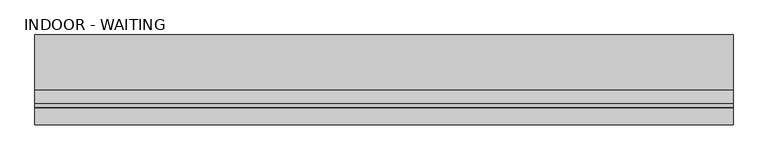
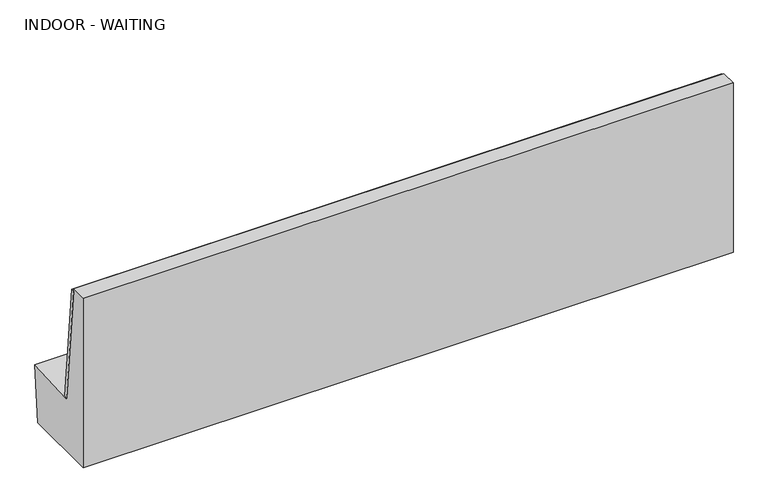
"""IFC4 building model written with IfcOpenShell, lengths in millimetres: furniture geometry, OD_CW_Booth : INDOOR - WAITING."""

from ifc_helpers import new_model, si_unit, frame, origin, place, context, project, spatial, polyline, outline, extrude, source, transform, mapped, element, save


def indoor_waiting_8bc71f9b(model_context):
    return source(origin(), model_context, "Body", "SweptSolid", [
        extrude(outline(polyline([(0.0, -5064.5281442), (0.0, 0.0), (25.4, 0.0), (25.4, -5064.5281442), (0.0, -5064.5281442)])), frame((5083.2658491, -358.2049359, 438.8309433), z_axis=(0.0, -0.10452846326765197, 0.9945218953682735), x_axis=(0.0, -0.9945218953682735, -0.10452846326765197)), (0.0, 0.0, 1.0), 944.7333479),
        extrude(outline(polyline([(-609.6, 1397.0), (-484.4524721, 1397.0), (-382.9385128, 431.1591941), (43.0849153, 453.4861359), (3.4100193, 0.0), (-609.6, 0.0), (-609.6, 1397.0)])), frame((18.7377049, 0.0, 0.0), z_axis=(1.0, 0.0, 0.0), x_axis=(0.0, 1.0, 0.0)), (0.0, 0.0, 1.0), 5064.5281442),
    ])


if __name__ == "__main__":
    model = new_model("IFC4")
    model_context = context("Model", 3, world=origin())
    ifc_project = project(units=[si_unit("LENGTHUNIT", "METRE", prefix="MILLI")], contexts=[model_context])
    site = spatial("IfcSite", under=ifc_project)
    building = spatial("IfcBuilding", under=site)
    placement = place(None, origin())
    indoor_waiting_shape = indoor_waiting_8bc71f9b(model_context)
    element("IfcFurniture", 1, ObjectType="OD_CW_Booth : INDOOR - WAITING", at=placement, inside=building, context=model_context, shape_type="MappedRepresentation", body=[
        mapped(indoor_waiting_shape, transform((0.0, 0.0, 0.0), x_axis=(1.0, 0.0, 0.0), y_axis=(0.0, 1.0, 0.0), z_axis=(0.0, 0.0, 1.0))),
    ])
    save(model, "model.ifc")

# Revit data of these elements
# Type "OD_CW_Booth : INDOOR - WAITING"
#   Width = 4' - 0"
#   OD_CW_Width [instance default] = 2' - 10"
#   OD_CW_Length [instance default] = 26' - 1 83/256"
#   OD_CW_Height [instance default] = 2' - 3"
#   Height = 3' - 0"
#   Depth = 2' - 0"
#   Seating Count [instance default] = 10
#   back = Casework-oakfire
#   OD_CW_Material_Front Panel [instance default] = none
#   OD_CW_Material_Body [instance default] = none
# Element 1 (IfcFurniture, "OD_CW_Booth : INDOOR - WAITING")
#   OD_CW_Length = 16' - 7.39087"
#   Seating Count = 6
#   OD_CW_Material_Body = WOOD-OAKFIRE
#   Materials on its faces: "WOOD-OAKFIRE", "Casework-oakfire"
# Materials
#   "Casework-oakfire": class "Miscellaneous", colour RGB 164 164 164, transparency 0, Cost = 0
#   "WOOD-OAKFIRE": class "Wood", colour RGB 198 202 183, transparency 0, Description = "Generic wood", Cost = 0
